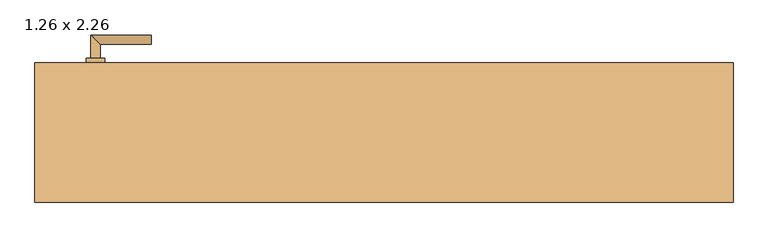
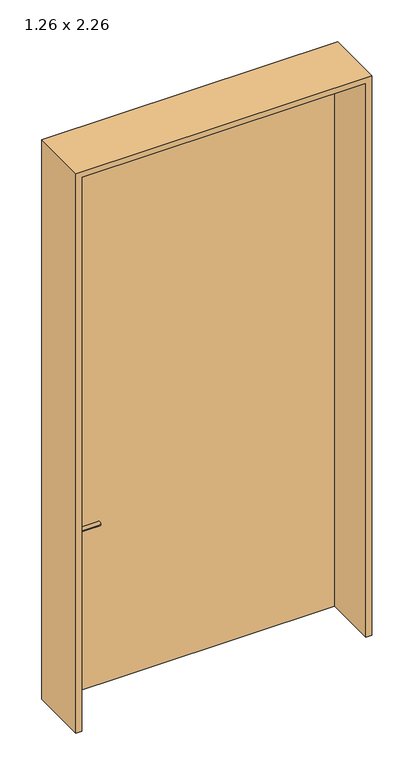
"""IFC4 building model written with IfcOpenShell, lengths in millimetres: door geometry, Drehflügel 1-flg - Blockzarge : 1.26 x 2.26."""

from ifc_helpers import new_model, si_unit, point, frame, frame_2d, origin, place, context, project, spatial, polyline, circle_curve, ellipse_curve, trimmed, segment, composite_curve, outline, extrude, source, transform, mapped, element, save
from ifc_brep_helpers import plane_surface, cylinder_surface, advanced_brep


def door_1_26_x_2_26_80e47a7c(model_context):
    return source(origin(), model_context, "Body", "SolidModel", [
        advanced_brep(
        [(-610.0, 129.4346141, 1000.0), (-630.0, 129.4346141, 1000.0), (-610.0, 99.4346141, 1000.0), (-630.0, 79.4346141, 1000.0), (-500.0, 99.4346141, 1000.0), (-500.0, 79.4346141, 1000.0)],
        [
            (0, 1, circle_curve(frame((-620.0, 129.4346141, 1000.0), z_axis=(0.0, 1.0, 0.0), x_axis=(-1.0, 0.0, 0.0)), 10.0)),
            (1, 0, circle_curve(frame((-620.0, 129.4346141, 1000.0), z_axis=(0.0, 1.0, 0.0), x_axis=(-1.0, 0.0, 0.0)), 10.0)),
            (0, 2),
            (2, 3, ellipse_curve(frame((-620.0, 89.4346141, 1000.0), z_axis=(-0.7071067811865686, 0.7071067811865265, 0.0), x_axis=(0.7071067811865264, 0.7071067811865687, 0.0)), 14.1421356, 10.0)),
            (3, 1),
            (3, 2, ellipse_curve(frame((-620.0, 89.4346141, 1000.0), z_axis=(-0.7071067811865686, 0.7071067811865265, 0.0), x_axis=(0.7071067811865264, 0.7071067811865687, 0.0)), 14.1421356, 10.0)),
            (4, 5, circle_curve(frame((-500.0, 89.4346141, 1000.0), z_axis=(1.0, 0.0, 0.0), x_axis=(0.0, -1.0, 0.0)), 10.0)),
            (5, 4, circle_curve(frame((-500.0, 89.4346141, 1000.0), z_axis=(1.0, 0.0, 0.0), x_axis=(0.0, -1.0, 0.0)), 10.0)),
            (2, 4),
            (5, 3),
        ],
        [
            plane_surface(frame((-620.0, 129.4346141, -287.7526403), z_axis=(0.0, 1.0, 0.0), x_axis=(0.0, 0.0, 1.0))),
            cylinder_surface(frame((-620.0, 129.4346141, 1000.0), z_axis=(0.0, 1.0, 0.0), x_axis=(-1.0, 0.0, 0.0)), 10.0),
            plane_surface(frame((-500.0, 89.4346141, -287.7526403), z_axis=(1.0, 0.0, 0.0), x_axis=(0.0, 0.0, 1.0))),
            cylinder_surface(frame((-620.0, 89.4346141, 1000.0), z_axis=(-1.0, 0.0, 0.0), x_axis=(0.0, -1.0, 0.0)), 10.0),
        ],
        [
            (0, [[1, 2]]),
            (1, [[-1, 3, 4, 5]]),
            (1, [[-2, -5, 6, -3]]),
            (2, [[7, 8]]),
            (3, [[-4, 9, -8, 10]]),
            (3, [[-6, -10, -7, -9]]),
        ],
    ),
        advanced_brep(
        [(-610.0, 174.4346141, 1000.0), (-630.0, 174.4346141, 1000.0), (-610.0, 204.4346141, 1000.0), (-630.0, 224.4346141, 1000.0), (-500.0, 204.4346141, 1000.0), (-500.0, 224.4346141, 1000.0)],
        [
            (0, 1, circle_curve(frame((-620.0, 174.4346141, 1000.0), z_axis=(0.0, -1.0, 0.0), x_axis=(-1.0, 0.0, 0.0)), 10.0)),
            (1, 0, circle_curve(frame((-620.0, 174.4346141, 1000.0), z_axis=(0.0, -1.0, 0.0), x_axis=(-1.0, 0.0, 0.0)), 10.0)),
            (0, 2),
            (2, 3, ellipse_curve(frame((-620.0, 214.4346141, 1000.0), z_axis=(-0.7071067811865486, -0.7071067811865464, 0.0), x_axis=(0.7071067811865464, -0.7071067811865488, 0.0)), 14.1421356, 10.0)),
            (3, 1),
            (3, 2, ellipse_curve(frame((-620.0, 214.4346141, 1000.0), z_axis=(-0.7071067811865486, -0.7071067811865464, 0.0), x_axis=(0.7071067811865464, -0.7071067811865488, 0.0)), 14.1421356, 10.0)),
            (4, 5, circle_curve(frame((-500.0, 214.4346141, 1000.0), z_axis=(1.0, 0.0, 0.0), x_axis=(0.0, 1.0, 0.0)), 10.0)),
            (5, 4, circle_curve(frame((-500.0, 214.4346141, 1000.0), z_axis=(1.0, 0.0, 0.0), x_axis=(0.0, 1.0, 0.0)), 10.0)),
            (2, 4),
            (5, 3),
        ],
        [
            plane_surface(frame((-620.0, 174.4346141, -287.7526403), z_axis=(0.0, -1.0, 0.0), x_axis=(0.0, 0.0, 1.0))),
            cylinder_surface(frame((-620.0, 174.4346141, 1000.0), z_axis=(0.0, -1.0, 0.0), x_axis=(-1.0, 0.0, 0.0)), 10.0),
            plane_surface(frame((-500.0, 214.4346141, -287.7526403), z_axis=(1.0, 0.0, 0.0), x_axis=(0.0, 0.0, 1.0))),
            cylinder_surface(frame((-620.0, 214.4346141, 1000.0), z_axis=(-1.0, 0.0, 0.0), x_axis=(0.0, 1.0, 0.0)), 10.0),
        ],
        [
            (0, [[1, 2]]),
            (1, [[-1, 3, 4, 5]]),
            (1, [[-2, -5, 6, -3]]),
            (2, [[7, 8]]),
            (3, [[-4, 9, -8, 10]]),
            (3, [[-6, -10, -7, -9]]),
        ],
    ),
        extrude(outline(composite_curve([segment(trimmed(circle_curve(frame_2d((1000.0, -620.0)), 20.0), [point((1000.0, -600.0))], [point((1000.0, -640.0))], False, "CARTESIAN"), True, "CONTINUOUS"), segment(trimmed(circle_curve(frame_2d((1000.0, -620.0)), 20.0), [point((1000.0, -640.0))], [point((1000.0, -600.0))], False, "CARTESIAN"), True, "CONTINUOUS")], self_intersect=False)), frame((0.0, 129.4346141, 0.0), z_axis=(0.0, 1.0, 0.0), x_axis=(0.0, 0.0, 1.0)), (0.0, 0.0, 1.0), 10.0),
        extrude(outline(composite_curve([segment(trimmed(circle_curve(frame_2d((1000.0, -620.0)), 20.0), [point((1000.0, -600.0))], [point((1000.0, -640.0))], False, "CARTESIAN"), True, "CONTINUOUS"), segment(trimmed(circle_curve(frame_2d((1000.0, -620.0)), 20.0), [point((1000.0, -640.0))], [point((1000.0, -600.0))], False, "CARTESIAN"), True, "CONTINUOUS")], self_intersect=False)), frame((0.0, 164.4346141, 0.0), z_axis=(0.0, 1.0, 0.0), x_axis=(0.0, 0.0, 1.0)), (0.0, 0.0, 1.0), 10.0),
        extrude(outline(polyline([(3100.0, 750.0), (3100.0, -750.0), (100.0, -750.0), (100.0, -720.0), (3070.0, -720.0), (3070.0, 720.0), (100.0, 720.0), (100.0, 750.0), (3100.0, 750.0)])), frame((0.0, -135.5653859, 0.0), z_axis=(0.0, 1.0, 0.0), x_axis=(0.0, 0.0, 1.0)), (0.0, 0.0, 1.0), 300.0),
        extrude(outline(polyline([(720.0, 164.4346141), (720.0, 139.4346141), (-720.0, 139.4346141), (-720.0, 164.4346141), (720.0, 164.4346141)])), frame((0.0, 0.0, 100.0), z_axis=(0.0, 0.0, 1.0), x_axis=(1.0, 0.0, 0.0)), (0.0, 0.0, 1.0), 2970.0),
    ])


if __name__ == "__main__":
    model = new_model("IFC4")
    model_context = context("Model", 3, world=origin())
    ifc_project = project(units=[si_unit("LENGTHUNIT", "METRE", prefix="MILLI")], contexts=[model_context])
    site = spatial("IfcSite", under=ifc_project)
    building = spatial("IfcBuilding", under=site)
    placement = place(None, origin())
    door_1_26_x_2_26_shape = door_1_26_x_2_26_80e47a7c(model_context)
    element("IfcDoor", 1, ObjectType="Drehflügel 1-flg - Blockzarge : 1.26 x 2.26", at=placement, inside=building, context=model_context, shape_type="MappedRepresentation", body=[
        mapped(door_1_26_x_2_26_shape, transform((0.0, 0.0, 0.0), x_axis=(1.0, 0.0, 0.0), y_axis=(0.0, 1.0, 0.0), z_axis=(0.0, 0.0, 1.0))),
    ])
    save(model, "model.ifc")

# Revit data of these elements
# Type "Drehflügel 1-flg - Blockzarge : 1.26 x 2.26"
#   Type Mark = "23"
#   Operation = "SingleSwingRight"
#   Keynote = "16.03"
#   Visual Light Transmittance = 0.9
#   Solar Heat Gain Coefficient = 0.86
#   Heat Transfer Coefficient (U) = 5.5617 W/(m²·K)
#   Rough Width = 1.500 m
#   Stärke Futter = 0.030 m
#   Rough Height [instance default] = 3.100 m
#   Höhe Türgriff = 0.900 m
#   Height = 3.000 m
#   Fußbodenaufbau [instance default] = 0.100 m
#   Width = 1.500 m
#   Sichtbarkeit Sturzlinien [instance default] = yes
#   Türgriff auswählen [instance default] = element 534090
#   Türgriff [instance default] = none
#   Türflügel [instance default] = none
#   Rahmen/Pfosten [instance default] = none
#   Construction Type Id = ""
#   Function = (empty or 0)
#   Wall Closure = (empty or 0)
#   Analytic Construction = (empty or 0)
# Element 1 (IfcDoor, "Drehflügel 1-flg - Blockzarge : 1.26 x 2.26")
#   Materials on its faces: "Metall - Chrom", "Holz - Birke"
# Materials
#   "Metall - Chrom": class "Metall", colour RGB 247 247 247, transparency 0, Cost = 0
#   "Holz - Birke": class "Holz", colour RGB 213 164 103, transparency 0, Cost = 0
